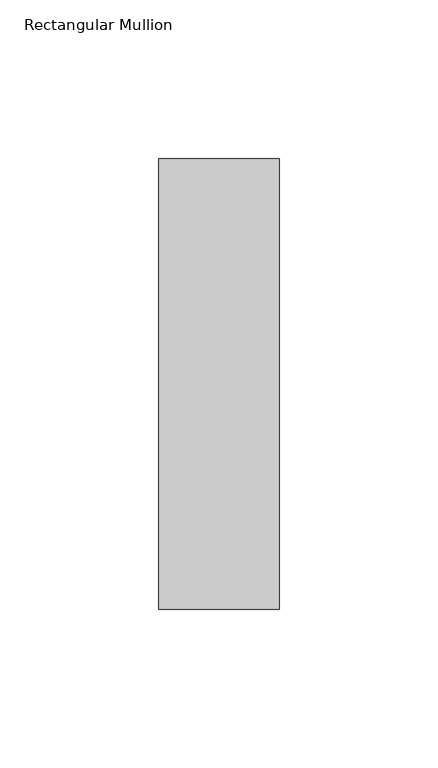
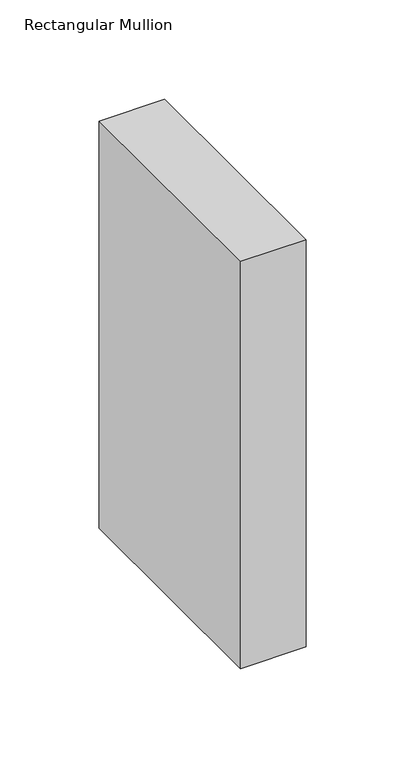
"""IFC4 building model written with IfcOpenShell, lengths in millimetres: member geometry, Rectangular Mullion : NLRS_21_CWM_hsb-regel 38x142_gen_rsf."""

from ifc_helpers import new_model, si_unit, frame, origin, place, context, project, spatial, polyline, outline, extrude, source, transform, mapped, element, save


def rectangular_mullion_56763ec6(model_context):
    return source(origin(), model_context, "Body", "SweptSolid", [
        extrude(outline(polyline([(-38.0, -71.0), (-38.0, 71.0), (0.0, 71.0), (0.0, -71.0), (-38.0, -71.0)])), frame((0.0, 0.0, -250.0000003), z_axis=(0.0, 0.0, 1.0), x_axis=(1.0, 0.0, 0.0)), (0.0, 0.0, 1.0), 250.0000003),
    ])


if __name__ == "__main__":
    model = new_model("IFC4")
    model_context = context("Model", 3, world=origin())
    ifc_project = project(units=[si_unit("LENGTHUNIT", "METRE", prefix="MILLI")], contexts=[model_context])
    site = spatial("IfcSite", under=ifc_project)
    building = spatial("IfcBuilding", under=site)
    placement = place(None, origin())
    rectangular_mullion_shape = rectangular_mullion_56763ec6(model_context)
    element("IfcMember", 1, ObjectType="Rectangular Mullion : NLRS_21_CWM_hsb-regel 38x142_gen_rsf", at=placement, inside=building, context=model_context, shape_type="MappedRepresentation", body=[
        mapped(rectangular_mullion_shape, transform((0.0, 0.0, 0.0), x_axis=(1.0, 0.0, 0.0), y_axis=(0.0, 1.0, 0.0), z_axis=(0.0, 0.0, 1.0))),
    ])
    save(model, "model.ifc")

# Revit data of these elements
# Type "Rectangular Mullion : NLRS_21_CWM_hsb-regel 38x142_gen_rsf"
#   Export Type to IFC As = "IfcWall"
#   Type IfcGUID = "07M7mRoiH1CR8m_RSKIwpF"
#   Assembly Code = "21.10"
#   built-in parameter 1007322 = 0.465879 (stored number, unit not read)
#   built-in parameter 1007321 = 0.062336 (stored number, unit not read)
#   built-in parameter 1007320 = 0.062336 (stored number, unit not read)
# Element 1 (IfcMember, "Rectangular Mullion : NLRS_21_CWM_hsb-regel 38x142_gen_rsf")
#   Materials on its faces: "NLRS_i2_hout naaldhout vuren_gen_rsf"
# Materials
#   "NLRS_i2_hout naaldhout vuren_gen_rsf": class "I - Hout", colour RGB 234 199 147, transparency 0, Keynote = "i2", Manufacturer = "Revit Standards Foundation", URL = "www.revitstandards.org", Description = "hout vuren", Cost = 0
